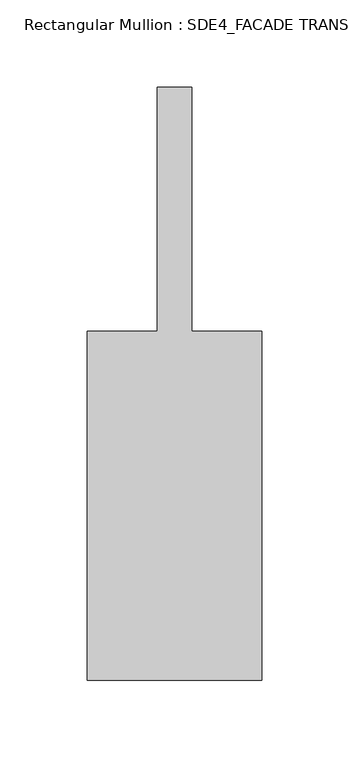
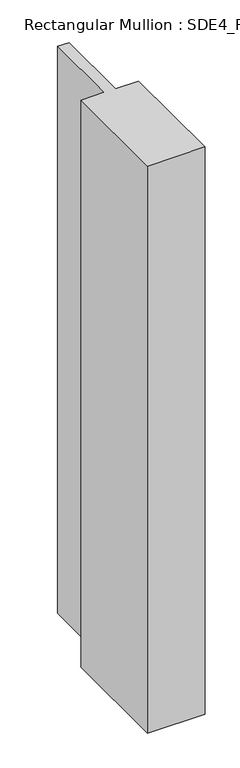
"""IFC4 building model written with IfcOpenShell, lengths in millimetres: member geometry, Rectangular Mullion : SDE4_FACADE TRANSOM TYPE 1."""

from ifc_helpers import new_model, si_unit, frame, origin, place, context, project, spatial, polyline, outline, extrude, source, transform, mapped, element, save


def rectangular_mullion_sde4_facade_transom_type_1_4372d292(model_context):
    return source(origin(), model_context, "Body", "SweptSolid", [
        extrude(outline(polyline([(50.0, -132.5), (-50.0, -132.5), (-50.0, 67.5), (-10.0, 67.5), (-10.0, 207.5), (10.0, 207.5), (10.0, 67.5), (50.0, 67.5), (50.0, -132.5)])), frame((0.0, 0.0, -1043.0375289), z_axis=(0.0, 0.0, 1.0), x_axis=(1.0, 0.0, 0.0)), (0.0, 0.0, 1.0), 1043.0375289),
    ])


if __name__ == "__main__":
    model = new_model("IFC4")
    model_context = context("Model", 3, world=origin())
    ifc_project = project(units=[si_unit("LENGTHUNIT", "METRE", prefix="MILLI")], contexts=[model_context])
    site = spatial("IfcSite", under=ifc_project)
    building = spatial("IfcBuilding", under=site)
    placement = place(None, origin())
    rectangular_mullion_sde4_facade_transom_type_1_shape = rectangular_mullion_sde4_facade_transom_type_1_4372d292(model_context)
    element("IfcMember", 1, ObjectType="Rectangular Mullion : SDE4_FACADE TRANSOM TYPE 1", at=placement, inside=building, context=model_context, shape_type="MappedRepresentation", body=[
        mapped(rectangular_mullion_sde4_facade_transom_type_1_shape, transform((0.0, 0.0, 0.0), x_axis=(1.0, 0.0, 0.0), y_axis=(0.0, 1.0, 0.0), z_axis=(0.0, 0.0, 1.0))),
    ])
    save(model, "model.ifc")

# Revit data of these elements
# Type "Rectangular Mullion : SDE4_FACADE TRANSOM TYPE 1"
#   built-in parameter 1007322 = 1.11549 (stored number, unit not read)
#   built-in parameter 1007321 = 0.164042 (stored number, unit not read)
#   built-in parameter 1007320 = 0.164042 (stored number, unit not read)
